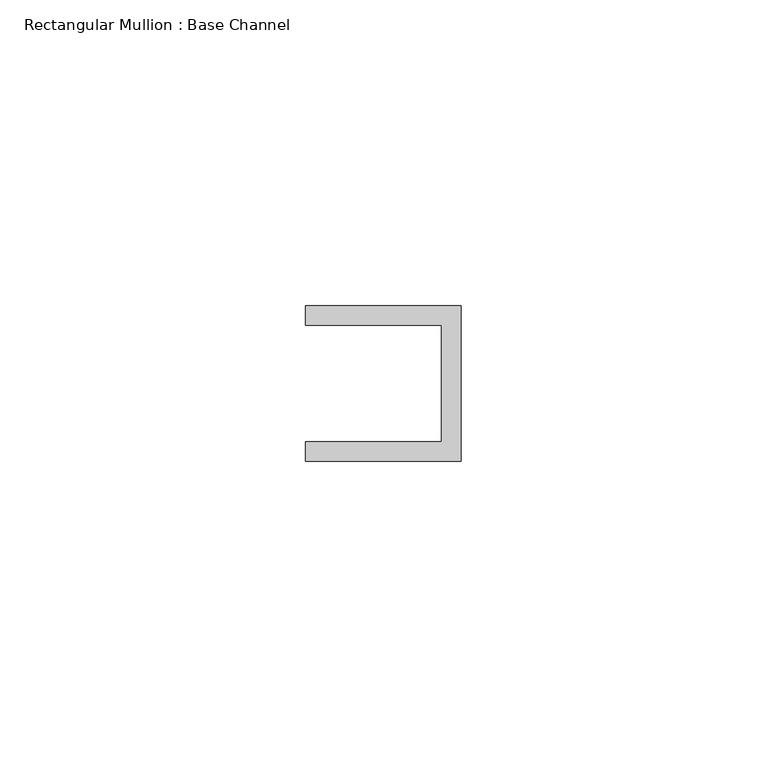
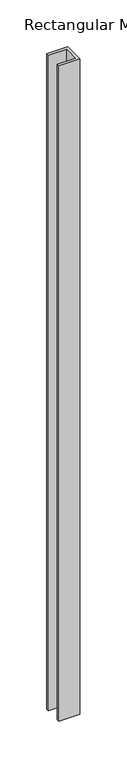
"""IFC4 building model written with IfcOpenShell, lengths in millimetres: member geometry, Rectangular Mullion : Base Channel."""

from ifc_helpers import new_model, si_unit, frame, origin, place, context, project, spatial, polyline, outline, extrude, source, transform, mapped, element, save


def rectangular_mullion_base_channel_d7a1e3f6(model_context):
    return source(origin(), model_context, "Body", "SweptSolid", [
        extrude(outline(polyline([(0.0, -12.7), (-25.4, -12.7), (-25.4, -9.525), (-3.175, -9.525), (-3.175, 9.525), (-25.4, 9.525), (-25.4, 12.7), (0.0, 12.7), (0.0, -12.7)])), frame((0.0, 0.0, -851.1267857), z_axis=(0.0, 0.0, 1.0), x_axis=(1.0, 0.0, 0.0)), (0.0, 0.0, 1.0), 851.1267857),
    ])


if __name__ == "__main__":
    model = new_model("IFC4")
    model_context = context("Model", 3, world=origin())
    ifc_project = project(units=[si_unit("LENGTHUNIT", "METRE", prefix="MILLI")], contexts=[model_context])
    site = spatial("IfcSite", under=ifc_project)
    building = spatial("IfcBuilding", under=site)
    placement = place(None, origin())
    rectangular_mullion_base_channel_shape = rectangular_mullion_base_channel_d7a1e3f6(model_context)
    element("IfcMember", 1, ObjectType="Rectangular Mullion : Base Channel", at=placement, inside=building, context=model_context, shape_type="MappedRepresentation", body=[
        mapped(rectangular_mullion_base_channel_shape, transform((0.0, 0.0, 0.0), x_axis=(1.0, 0.0, 0.0), y_axis=(0.0, 1.0, 0.0), z_axis=(0.0, 0.0, 1.0))),
    ])
    save(model, "model.ifc")

# Revit data of these elements
# Type "Rectangular Mullion : Base Channel"
#   built-in parameter 1007322 = 0.0833333 (stored number, unit not read)
#   built-in parameter 1007321 = 0.0416667 (stored number, unit not read)
#   built-in parameter 1007320 = -0.03125 (stored number, unit not read)
# Element 1 (IfcMember, "Rectangular Mullion : Base Channel")
#   Materials on its faces: "ALUM"
# Materials
#   "ALUM": class "Generic", colour RGB 157 157 157, transparency 0, Cost = 0
